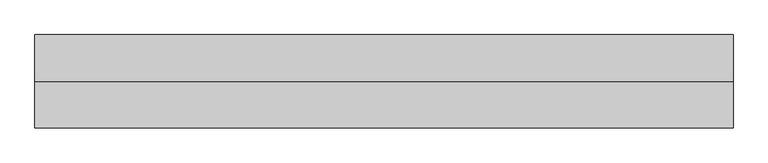
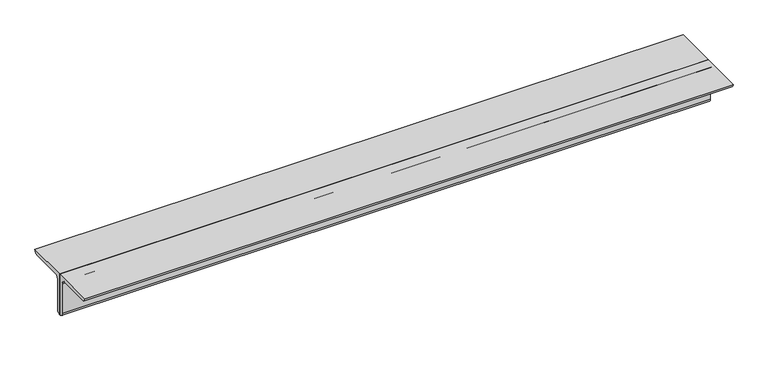
"""IFC4 building model written with IfcOpenShell, lengths in millimetres: beam geometry, 0123_Steel Framing_2Ls-KSD3502 : H_SB_AR_S04_2Ls-130x130x12_VBR1."""

import ifcopenshell
import ifcopenshell.guid

model = None  # the IFC model being written
_history = None  # IfcOwnerHistory: only IFC2X3 demands one
_inside = {}  # id of a spatial element -> (the spatial element, [elements in it])
_under = {}  # id of a project, library or spatial element -> (it, [spatial elements below it])
_declared = {}  # id of a project -> (the project, [libraries it declares])
_typed = {}  # id of a type object -> (the type object, [elements of that type])
_made_of = {}  # id of a material, layer set ... -> (it, [elements and type objects made of it])


def new_model(schema):
    """Start an empty IFC model of exactly this schema.

    Asked for "IFC4X3", IfcOpenShell would pick the latest addendum, in which some entities
    have other attributes; the version numbers below select the first issue.
    IFC2X3 requires an IfcOwnerHistory on every rooted entity: one is made here for all.
    """
    global model, _history
    if schema == "IFC4X3":
        model = ifcopenshell.file(schema_version=(4, 3, 0, 0))
    else:
        model = ifcopenshell.file(schema=schema)
    _inside.clear()
    _under.clear()
    _declared.clear()
    _typed.clear()
    _made_of.clear()
    _history = None
    if model.schema == "IFC2X3":
        org = make("IfcOrganization", Name="unknown")
        user = make(
            "IfcPersonAndOrganization",
            ThePerson=make("IfcPerson", FamilyName="unknown"),
            TheOrganization=org,
        )
        app = make(
            "IfcApplication",
            ApplicationDeveloper=org,
            Version="unknown",
            ApplicationFullName="unknown",
            ApplicationIdentifier="unknown",
        )
        _history = make(
            "IfcOwnerHistory",
            OwningUser=user,
            OwningApplication=app,
            ChangeAction="ADDED",
            CreationDate=0,
        )
    return model


def make(cls, **values):
    """One entity of the class cls with the attributes given. An attribute that is None is left unset."""
    return model.create_entity(
        cls, **{name: value for name, value in values.items() if value is not None}
    )


def rooted(cls, **values):
    """An entity with a GlobalId (a new one), such as an element, a storey or a relation."""
    return make(cls, GlobalId=ifcopenshell.guid.new(), OwnerHistory=_history, **values)


def si_unit(unit_type, name, prefix=None):
    """IfcSIUnit, for example si_unit("LENGTHUNIT", "METRE", prefix="MILLI")."""
    return make("IfcSIUnit", UnitType=unit_type, Prefix=prefix, Name=name)


def assignment(units):
    """IfcUnitAssignment: the units of a project."""
    return None if units is None else make("IfcUnitAssignment", Units=units)


def point(xyz):
    """IfcCartesianPoint."""
    return None if xyz is None else make("IfcCartesianPoint", Coordinates=xyz)


def direction(xyz):
    """IfcDirection."""
    return None if xyz is None else make("IfcDirection", DirectionRatios=xyz)


def frame(location, z_axis=None, x_axis=None):
    """IfcAxis2Placement3D, a coordinate frame: its origin and axes. An axis left out is left unset."""
    return make(
        "IfcAxis2Placement3D",
        Location=point(location),
        Axis=direction(z_axis),
        RefDirection=direction(x_axis),
    )


def frame_2d(location, x_axis=None):
    """IfcAxis2Placement2D, a coordinate frame in the plane: its origin and x axis."""
    return make(
        "IfcAxis2Placement2D", Location=point(location), RefDirection=direction(x_axis)
    )


def origin():
    """The frame at (0, 0, 0) with its axes left unset."""
    return frame((0.0, 0.0, 0.0))


def place(relative_to, where):
    """IfcLocalPlacement: puts the frame where relative to a parent placement (None: the world)."""
    return make(
        "IfcLocalPlacement", PlacementRelTo=relative_to, RelativePlacement=where
    )


def context(
    kind, dimensions, precision=None, world=None, true_north=None, identifier=None
):
    """IfcGeometricRepresentationContext, for example the 3D "Model" context."""
    return make(
        "IfcGeometricRepresentationContext",
        ContextIdentifier=identifier,
        ContextType=kind,
        CoordinateSpaceDimension=dimensions,
        Precision=precision,
        WorldCoordinateSystem=world,
        TrueNorth=true_north,
    )


def project(units=None, contexts=None):
    """IfcProject with its units and contexts."""
    return rooted(
        "IfcProject",
        Name="project",
        RepresentationContexts=contexts,
        UnitsInContext=assignment(units),
    )


def spatial(cls, under=None, at=None, **own):
    """A site, building, storey or space (cls), placed at a placement, below another one or the project."""
    s = rooted(cls, ObjectPlacement=at, **own)
    if under is not None:
        _under.setdefault(under.id(), (under, []))[1].append(s)
    return s


def polyline(points):
    """IfcPolyline through the points."""
    return make("IfcPolyline", Points=[point(p) for p in points])


def circle_curve(where, radius):
    """IfcCircle in the frame where."""
    return make("IfcCircle", Position=where, Radius=radius)


def trimmed(basis, trim1, trim2, sense, master):
    """IfcTrimmedCurve: the piece of a basis curve between two trims."""
    return make(
        "IfcTrimmedCurve",
        BasisCurve=basis,
        Trim1=trim1,
        Trim2=trim2,
        SenseAgreement=sense,
        MasterRepresentation=master,
    )


def segment(curve, same_sense, transition):
    """IfcCompositeCurveSegment."""
    return make(
        "IfcCompositeCurveSegment",
        Transition=transition,
        SameSense=same_sense,
        ParentCurve=curve,
    )


def composite_curve(segments, self_intersect=None):
    """IfcCompositeCurve: segments joined end to end."""
    return make("IfcCompositeCurve", Segments=segments, SelfIntersect=self_intersect)


def outline(outer, holes=None, kind="AREA"):
    """IfcArbitraryClosedProfileDef: a profile drawn as a closed curve; with holes, ...WithVoids."""
    if holes is None:
        return make("IfcArbitraryClosedProfileDef", ProfileType=kind, OuterCurve=outer)
    return make(
        "IfcArbitraryProfileDefWithVoids",
        ProfileType=kind,
        OuterCurve=outer,
        InnerCurves=holes,
    )


def extrude(swept, where, along, depth):
    """IfcExtrudedAreaSolid: the profile swept, set in the frame where, extruded along a direction by depth."""
    return make(
        "IfcExtrudedAreaSolid",
        SweptArea=swept,
        Position=where,
        ExtrudedDirection=direction(along),
        Depth=depth,
    )


def shape(context_of_items, identifier, shape_type, items):
    """IfcShapeRepresentation: the items that make up one representation, for example the "Body"."""
    return make(
        "IfcShapeRepresentation",
        ContextOfItems=context_of_items,
        RepresentationIdentifier=identifier,
        RepresentationType=shape_type,
        Items=items,
    )


def source(mapping_origin, context_of_items, identifier, shape_type, items):
    """IfcRepresentationMap: a shape defined once, which mapped items show again and again."""
    return make(
        "IfcRepresentationMap",
        MappingOrigin=mapping_origin,
        MappedRepresentation=shape(context_of_items, identifier, shape_type, items),
    )


def transform(
    local_origin,
    x_axis=None,
    y_axis=None,
    z_axis=None,
    scale=None,
    scale2=None,
    scale3=None,
    uniform=True,
):
    """IfcCartesianTransformationOperator3D, or its non-uniform kind. x_axis, y_axis, z_axis: its Axis1, 2, 3."""
    if uniform:
        return make(
            "IfcCartesianTransformationOperator3D",
            Axis1=direction(x_axis),
            Axis2=direction(y_axis),
            LocalOrigin=point(local_origin),
            Scale=scale,
            Axis3=direction(z_axis),
        )
    return make(
        "IfcCartesianTransformationOperator3DnonUniform",
        Axis1=direction(x_axis),
        Axis2=direction(y_axis),
        LocalOrigin=point(local_origin),
        Scale=scale,
        Axis3=direction(z_axis),
        Scale2=scale2,
        Scale3=scale3,
    )


def mapped(mapping_source, mapping_target):
    """IfcMappedItem: shows the shape of a source again, moved by a transform."""
    return make(
        "IfcMappedItem", MappingSource=mapping_source, MappingTarget=mapping_target
    )


def made_of(thing, what):
    """Note that an element or type object is made of a material, layer set ...; save() writes the relation."""
    if what is not None:
        _made_of.setdefault(what.id(), (what, []))[1].append(thing)
    return thing


def element(
    cls,
    number,
    at=None,
    inside=None,
    cuts=None,
    type_object=None,
    material=None,
    context=None,
    identifier="Body",
    shape_type=None,
    held_by="IfcProductDefinitionShape",
    body=None,
    shapes=None,
    **own,
):
    """One element of the class cls, such as IfcWall. Its Tag is "e" and its number.

    at: its placement. inside: the storey or other place that contains it. cuts: it is an
    opening in that element (IfcRelVoidsElement). A single representation is given by context,
    identifier, shape_type and body (its items); several are given by shapes. held_by: the class
    of the entity that holds the representations. save() writes the other relations.
    """
    e = rooted(cls, Tag="e%d" % number, ObjectPlacement=at, **own)
    if body is not None:
        shapes = [shape(context, identifier, shape_type, body)]
    if shapes is not None:
        e.Representation = make(held_by, Representations=shapes)
    if inside is not None:
        _inside.setdefault(inside.id(), (inside, []))[1].append(e)
    if cuts is not None:
        rooted(
            "IfcRelVoidsElement", RelatingBuildingElement=cuts, RelatedOpeningElement=e
        )
    if type_object is not None:
        _typed.setdefault(type_object.id(), (type_object, []))[1].append(e)
    return made_of(e, material)


def aggregate(whole, parts):
    """IfcRelAggregates: a whole, such as a stair, and the parts it consists of."""
    return rooted("IfcRelAggregates", RelatingObject=whole, RelatedObjects=parts)


def save(model, path):
    """Write the relations noted so far, then the file.

    IfcRelAggregates (storeys below a building ...), IfcRelContainedInSpatialStructure (elements
    in a storey), IfcRelDefinesByType, IfcRelAssociatesMaterial and IfcRelDeclares: one each for
    every whole, place, type object, material and project.
    """
    for whole, parts in _under.values():
        aggregate(whole, parts)
    for where, things in _inside.values():
        rooted(
            "IfcRelContainedInSpatialStructure",
            RelatedElements=things,
            RelatingStructure=where,
        )
    for kind, things in _typed.values():
        rooted("IfcRelDefinesByType", RelatedObjects=things, RelatingType=kind)
    for what, things in _made_of.values():
        rooted("IfcRelAssociatesMaterial", RelatedObjects=things, RelatingMaterial=what)
    for by, libraries in _declared.values():
        rooted("IfcRelDeclares", RelatingContext=by, RelatedDefinitions=libraries)
    model.write(path)


def beam_4cc4f4f8(model_context):
    return source(origin(), model_context, "Body", "SweptSolid", [
        extrude(outline(composite_curve([segment(polyline([(0.0, 36.4), (130.0, 36.4)]), True, "CONTINUOUS"), segment(trimmed(circle_curve(frame_2d((118.0, 36.4)), 12.0), [point((130.0, 36.4))], [point((118.0, 24.4))], False, "CARTESIAN"), True, "CONTINUOUS"), segment(polyline([(118.0, 24.4), (24.0, 24.4)]), True, "CONTINUOUS"), segment(trimmed(circle_curve(frame_2d((24.0, 12.4)), 12.0), [point((24.0, 24.4))], [point((12.0, 12.4))], True, "CARTESIAN"), True, "CONTINUOUS"), segment(polyline([(12.0, 12.4), (12.0, -81.6)]), True, "CONTINUOUS"), segment(trimmed(circle_curve(frame_2d((0.0, -81.6)), 12.0), [point((12.0, -81.6))], [point((0.0, -93.6))], False, "CARTESIAN"), True, "CONTINUOUS"), segment(polyline([(0.0, -93.6), (0.0, 36.4)]), True, "CONTINUOUS")], self_intersect=False)), frame((-905.8182142, 0.0, 0.0), z_axis=(1.0, 0.0, 0.0), x_axis=(0.0, 1.0, 0.0)), (0.0, 0.0, 1.0), 1947.4481229),
        extrude(outline(composite_curve([segment(polyline([(0.0, 36.4), (0.0, -93.6)]), True, "CONTINUOUS"), segment(trimmed(circle_curve(frame_2d((0.0, -81.6)), 12.0), [point((0.0, -93.6))], [point((-12.0, -81.6))], False, "CARTESIAN"), True, "CONTINUOUS"), segment(polyline([(-12.0, -81.6), (-12.0, 12.4)]), True, "CONTINUOUS"), segment(trimmed(circle_curve(frame_2d((-24.0, 12.4)), 12.0), [point((-12.0, 12.4))], [point((-24.0, 24.4))], True, "CARTESIAN"), True, "CONTINUOUS"), segment(polyline([(-24.0, 24.4), (-118.0, 24.4)]), True, "CONTINUOUS"), segment(trimmed(circle_curve(frame_2d((-118.0, 36.4)), 12.0), [point((-118.0, 24.4))], [point((-130.0, 36.4))], False, "CARTESIAN"), True, "CONTINUOUS"), segment(polyline([(-130.0, 36.4), (0.0, 36.4)]), True, "CONTINUOUS")], self_intersect=False)), frame((-905.8182142, 0.0, 0.0), z_axis=(1.0, 0.0, 0.0), x_axis=(0.0, 1.0, 0.0)), (0.0, 0.0, 1.0), 1947.4481229),
    ])


if __name__ == "__main__":
    model = new_model("IFC4")
    model_context = context("Model", 3, world=origin())
    ifc_project = project(units=[si_unit("LENGTHUNIT", "METRE", prefix="MILLI")], contexts=[model_context])
    site = spatial("IfcSite", under=ifc_project)
    building = spatial("IfcBuilding", under=site)
    placement = place(None, origin())
    beam_shape = beam_4cc4f4f8(model_context)
    element("IfcBeam", 1, ObjectType="0123_Steel Framing_2Ls-KSD3502 : H_SB_AR_S04_2Ls-130x130x12_VBR1", at=placement, inside=building, context=model_context, shape_type="MappedRepresentation", body=[
        mapped(beam_shape, transform((0.0, 0.0, 0.0), x_axis=(1.0, 0.0, 0.0), y_axis=(0.0, 1.0, 0.0), z_axis=(0.0, 0.0, 1.0))),
    ])
    save(model, "model.ifc")

# Revit data of these elements
# Type "0123_Steel Framing_2Ls-KSD3502 : H_SB_AR_S04_2Ls-130x130x12_VBR1"
#   Type Mark = "VBR1"
#   Assembly Code = "B10"
#   Legs = "SLBB"
#   W = 8.97
#   Perimeter = 1.04 m²/m
#   Nominal Weight = 46.80 kgf/m
#   Length [instance default] = 1000 mm
#   Space = 0 mm
#   b = 130 mm
#   d = 130 mm
#   t = 12 mm
#   y = 36.4 mm
#   A = 0.005952 m²
#   Structural Material [instance default] = Steel ASTM A36
# Element 1 (IfcBeam, "0123_Steel Framing_2Ls-KSD3502 : H_SB_AR_S04_2Ls-130x130x12_VBR1")
#   Materials on its faces: "Steel ASTM A36"
# Materials
#   "Steel ASTM A36": class "Metal", colour RGB 199 199 199, transparency 0, Description = "Structural steel, ASTM A36 Grade B, mill finish", Cost = 0
